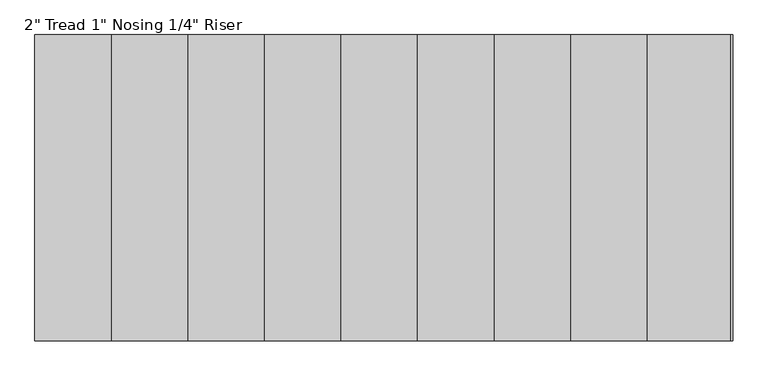
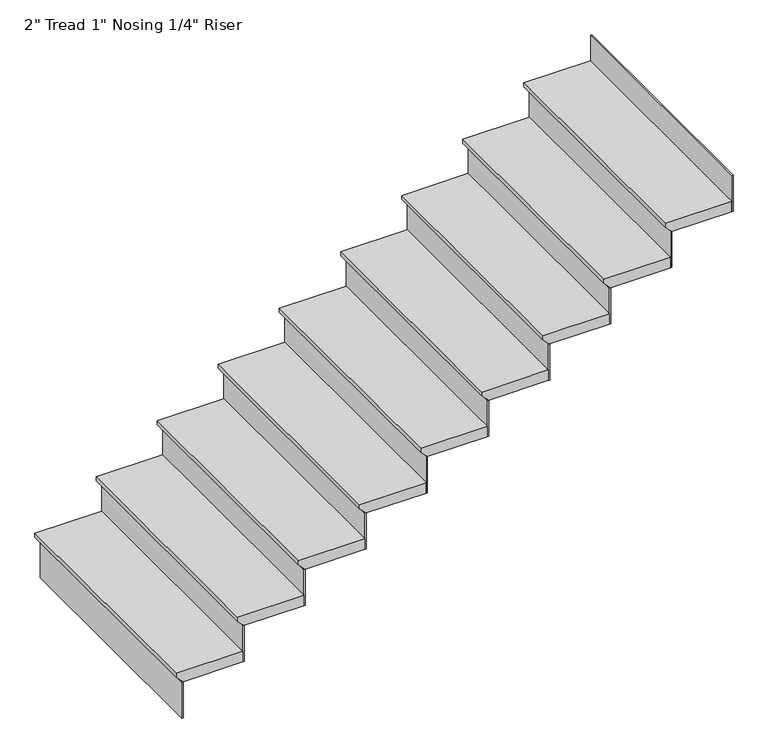
"""IFC4 building model written with IfcOpenShell, lengths in millimetres: stair flight geometry."""

from ifc_helpers import new_model, si_unit, frame, origin, place, context, project, spatial, polyline, outline, extrude, source, transform, mapped, element, save


def stair_flight_4c39f742(model_context):
    return source(origin(), model_context, "Body", "SweptSolid", [
        extrude(outline(polyline([(5747.6571429, -3197.8122732), (5747.6571429, -3502.6122732), (5728.6071429, -3502.6122732), (5703.2071429, -3477.2122732), (5696.8571429, -3477.2122732), (5696.8571429, -3197.8122732), (5747.6571429, -3197.8122732)])), frame((0.0, 8132.6265304, 0.0), z_axis=(0.0, 1.0, 0.0), x_axis=(0.0, 0.0, 1.0)), (0.0, 0.0, 1.0), 1117.6),
        extrude(outline(polyline([(-3470.8622732, 8132.6265304), (-3477.2122732, 8132.6265304), (-3477.2122732, 9250.2265304), (-3470.8622732, 9250.2265304), (-3470.8622732, 8132.6265304)])), frame((0.0, 0.0, 5522.6857143), z_axis=(0.0, 0.0, 1.0), x_axis=(1.0, 0.0, 0.0)), (0.0, 0.0, 1.0), 174.1714286),
        extrude(outline(polyline([(-3191.4622732, 8132.6265304), (-3197.8122732, 8132.6265304), (-3197.8122732, 9250.2265304), (-3191.4622732, 9250.2265304), (-3191.4622732, 8132.6265304)])), frame((0.0, 0.0, 5696.8571429), z_axis=(0.0, 0.0, 1.0), x_axis=(1.0, 0.0, 0.0)), (0.0, 0.0, 1.0), 174.1714286),
        extrude(outline(polyline([(5921.8285714, -2918.4122732), (5921.8285714, -3223.2122732), (5902.7785714, -3223.2122732), (5877.3785714, -3197.8122732), (5871.0285714, -3197.8122732), (5871.0285714, -2918.4122732), (5921.8285714, -2918.4122732)])), frame((0.0, 8132.6265304, 0.0), z_axis=(0.0, 1.0, 0.0), x_axis=(0.0, 0.0, 1.0)), (0.0, 0.0, 1.0), 1117.6),
        extrude(outline(polyline([(-2912.0622732, 8132.6265304), (-2918.4122732, 8132.6265304), (-2918.4122732, 9250.2265304), (-2912.0622732, 9250.2265304), (-2912.0622732, 8132.6265304)])), frame((0.0, 0.0, 5871.0285714), z_axis=(0.0, 0.0, 1.0), x_axis=(1.0, 0.0, 0.0)), (0.0, 0.0, 1.0), 174.1714286),
        extrude(outline(polyline([(6096.0, -2639.0122732), (6096.0, -2943.8122732), (6076.95, -2943.8122732), (6051.55, -2918.4122732), (6045.2, -2918.4122732), (6045.2, -2639.0122732), (6096.0, -2639.0122732)])), frame((0.0, 8132.6265304, 0.0), z_axis=(0.0, 1.0, 0.0), x_axis=(0.0, 0.0, 1.0)), (0.0, 0.0, 1.0), 1117.6),
        extrude(outline(polyline([(-2632.6622732, 8132.6265304), (-2639.0122732, 8132.6265304), (-2639.0122732, 9250.2265304), (-2632.6622732, 9250.2265304), (-2632.6622732, 8132.6265304)])), frame((0.0, 0.0, 6045.2), z_axis=(0.0, 0.0, 1.0), x_axis=(1.0, 0.0, 0.0)), (0.0, 0.0, 1.0), 174.1714286),
        extrude(outline(polyline([(6270.1714286, -2359.6122732), (6270.1714286, -2664.4122732), (6251.1214286, -2664.4122732), (6225.7214286, -2639.0122732), (6219.3714286, -2639.0122732), (6219.3714286, -2359.6122732), (6270.1714286, -2359.6122732)])), frame((0.0, 8132.6265304, 0.0), z_axis=(0.0, 1.0, 0.0), x_axis=(0.0, 0.0, 1.0)), (0.0, 0.0, 1.0), 1117.6),
        extrude(outline(polyline([(-2353.2622732, 8132.6265304), (-2359.6122732, 8132.6265304), (-2359.6122732, 9250.2265304), (-2353.2622732, 9250.2265304), (-2353.2622732, 8132.6265304)])), frame((0.0, 0.0, 6219.3714286), z_axis=(0.0, 0.0, 1.0), x_axis=(1.0, 0.0, 0.0)), (0.0, 0.0, 1.0), 174.1714286),
        extrude(outline(polyline([(6444.3428571, -2080.2122732), (6444.3428571, -2385.0122732), (6425.2928571, -2385.0122732), (6399.8928571, -2359.6122732), (6393.5428571, -2359.6122732), (6393.5428571, -2080.2122732), (6444.3428571, -2080.2122732)])), frame((0.0, 8132.6265304, 0.0), z_axis=(0.0, 1.0, 0.0), x_axis=(0.0, 0.0, 1.0)), (0.0, 0.0, 1.0), 1117.6),
        extrude(outline(polyline([(-2073.8622732, 8132.6265304), (-2080.2122732, 8132.6265304), (-2080.2122732, 9250.2265304), (-2073.8622732, 9250.2265304), (-2073.8622732, 8132.6265304)])), frame((0.0, 0.0, 6393.5428571), z_axis=(0.0, 0.0, 1.0), x_axis=(1.0, 0.0, 0.0)), (0.0, 0.0, 1.0), 174.1714286),
        extrude(outline(polyline([(6618.5142857, -1800.8122732), (6618.5142857, -2105.6122732), (6599.4642857, -2105.6122732), (6574.0642857, -2080.2122732), (6567.7142857, -2080.2122732), (6567.7142857, -1800.8122732), (6618.5142857, -1800.8122732)])), frame((0.0, 8132.6265304, 0.0), z_axis=(0.0, 1.0, 0.0), x_axis=(0.0, 0.0, 1.0)), (0.0, 0.0, 1.0), 1117.6),
        extrude(outline(polyline([(-1794.4622732, 8132.6265304), (-1800.8122732, 8132.6265304), (-1800.8122732, 9250.2265304), (-1794.4622732, 9250.2265304), (-1794.4622732, 8132.6265304)])), frame((0.0, 0.0, 6567.7142857), z_axis=(0.0, 0.0, 1.0), x_axis=(1.0, 0.0, 0.0)), (0.0, 0.0, 1.0), 174.1714286),
        extrude(outline(polyline([(6792.6857143, -1521.4122732), (6792.6857143, -1826.2122732), (6773.6357143, -1826.2122732), (6748.2357143, -1800.8122732), (6741.8857143, -1800.8122732), (6741.8857143, -1521.4122732), (6792.6857143, -1521.4122732)])), frame((0.0, 8132.6265304, 0.0), z_axis=(0.0, 1.0, 0.0), x_axis=(0.0, 0.0, 1.0)), (0.0, 0.0, 1.0), 1117.6),
        extrude(outline(polyline([(-1515.0622732, 8132.6265304), (-1521.4122732, 8132.6265304), (-1521.4122732, 9250.2265304), (-1515.0622732, 9250.2265304), (-1515.0622732, 8132.6265304)])), frame((0.0, 0.0, 6741.8857143), z_axis=(0.0, 0.0, 1.0), x_axis=(1.0, 0.0, 0.0)), (0.0, 0.0, 1.0), 174.1714286),
        extrude(outline(polyline([(6966.8571429, -1242.0122732), (6966.8571429, -1546.8122732), (6947.8071429, -1546.8122732), (6922.4071429, -1521.4122732), (6916.0571429, -1521.4122732), (6916.0571429, -1242.0122732), (6966.8571429, -1242.0122732)])), frame((0.0, 8132.6265304, 0.0), z_axis=(0.0, 1.0, 0.0), x_axis=(0.0, 0.0, 1.0)), (0.0, 0.0, 1.0), 1117.6),
        extrude(outline(polyline([(-1235.6622732, 8132.6265304), (-1242.0122732, 8132.6265304), (-1242.0122732, 9250.2265304), (-1235.6622732, 9250.2265304), (-1235.6622732, 8132.6265304)])), frame((0.0, 0.0, 6916.0571429), z_axis=(0.0, 0.0, 1.0), x_axis=(1.0, 0.0, 0.0)), (0.0, 0.0, 1.0), 174.1714286),
        extrude(outline(polyline([(-956.2622732, 8132.6265304), (-962.6122732, 8132.6265304), (-962.6122732, 9250.2265304), (-956.2622732, 9250.2265304), (-956.2622732, 8132.6265304)])), frame((0.0, 0.0, 7090.2285714), z_axis=(0.0, 0.0, 1.0), x_axis=(1.0, 0.0, 0.0)), (0.0, 0.0, 1.0), 174.1714286),
        extrude(outline(polyline([(7141.0285714, -962.6122732), (7141.0285714, -1267.4122732), (7121.9785714, -1267.4122732), (7096.5785714, -1242.0122732), (7090.2285714, -1242.0122732), (7090.2285714, -962.6122732), (7141.0285714, -962.6122732)])), frame((0.0, 8132.6265304, 0.0), z_axis=(0.0, 1.0, 0.0), x_axis=(0.0, 0.0, 1.0)), (0.0, 0.0, 1.0), 1117.6),
    ])


if __name__ == "__main__":
    model = new_model("IFC4")
    model_context = context("Model", 3, world=origin())
    ifc_project = project(units=[si_unit("LENGTHUNIT", "METRE", prefix="MILLI")], contexts=[model_context])
    site = spatial("IfcSite", under=ifc_project)
    building = spatial("IfcBuilding", under=site)
    placement = place(None, origin())
    stair_flight_shape = stair_flight_4c39f742(model_context)
    element("IfcStairFlight", 1, ObjectType="2\" Tread 1\" Nosing 1/4\" Riser", at=placement, inside=building, context=model_context, shape_type="MappedRepresentation", body=[
        mapped(stair_flight_shape, transform((0.0, 0.0, 0.0), x_axis=(1.0, 0.0, 0.0), y_axis=(0.0, 1.0, 0.0), z_axis=(0.0, 0.0, 1.0))),
    ])
    save(model, "model.ifc")
